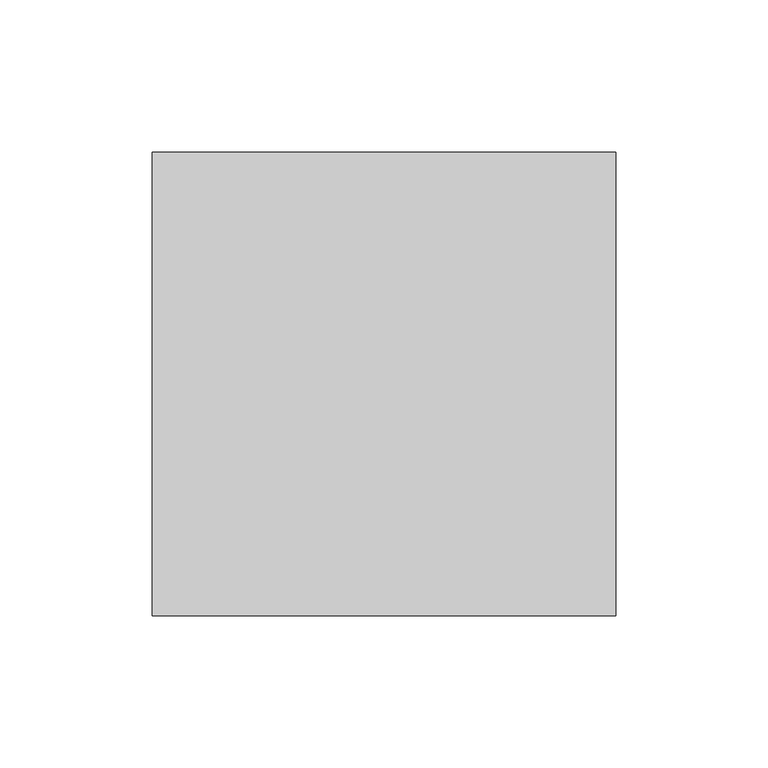
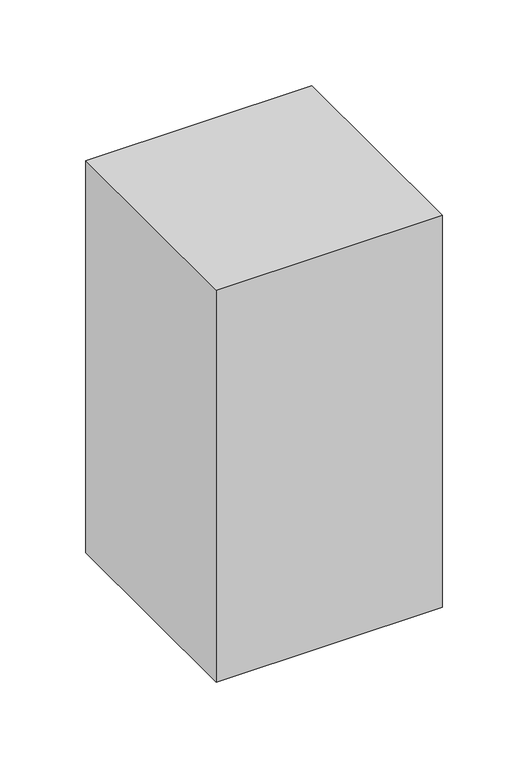
"""IFC4 building model written with IfcOpenShell, lengths in millimetres: proxy geometry, Seqm-Toilet Paper Disp-UH-3D : Seqm-Toilet Paper Disp-UH-3D."""

from ifc_helpers import new_model, si_unit, frame, origin, place, context, project, spatial, polyline, outline, extrude, source, transform, mapped, element, save


def specialty_equipment_997e0a6d(model_context):
    return source(origin(), model_context, "Body", "SweptSolid", [
        extrude(outline(polyline([(76.2, 0.0), (76.2, -152.4), (-76.2, -152.4), (-76.2, 0.0), (76.2, 0.0)])), frame((0.0, 0.0, 457.2), z_axis=(0.0, 0.0, 1.0), x_axis=(1.0, 0.0, 0.0)), (0.0, 0.0, 1.0), 279.4),
    ])


if __name__ == "__main__":
    model = new_model("IFC4")
    model_context = context("Model", 3, world=origin())
    ifc_project = project(units=[si_unit("LENGTHUNIT", "METRE", prefix="MILLI")], contexts=[model_context])
    site = spatial("IfcSite", under=ifc_project)
    building = spatial("IfcBuilding", under=site)
    placement = place(None, origin())
    specialty_equipment_shape = specialty_equipment_997e0a6d(model_context)
    element("IfcBuildingElementProxy", 1, Name="Seqm-Toilet Paper Disp-UH-3D : Seqm-Toilet Paper Disp-UH-3D", ObjectType="Seqm-Toilet Paper Disp-UH-3D : Seqm-Toilet Paper Disp-UH-3D", at=placement, inside=building, context=model_context, shape_type="MappedRepresentation", body=[
        mapped(specialty_equipment_shape, transform((0.0, 0.0, 0.0), x_axis=(1.0, 0.0, 0.0), y_axis=(0.0, 1.0, 0.0), z_axis=(0.0, 0.0, 1.0))),
    ])
    save(model, "model.ifc")

# Revit data of these elements
# Type "Seqm-Toilet Paper Disp-UH-3D : Seqm-Toilet Paper Disp-UH-3D"
#   Width = 0' - 6"
#   Height from Floor = 1' - 6"
#   Height = 0' - 11"
#   Depth = 0' - 6"
# Element 1 (IfcBuildingElementProxy, "Seqm-Toilet Paper Disp-UH-3D : Seqm-Toilet Paper Disp-UH-3D")
#   Materials on its faces: "TOILET PAPER DISPENSER"
# Materials
#   "TOILET PAPER DISPENSER": class "Generic", colour RGB 120 120 120, transparency 0, Cost = 0
